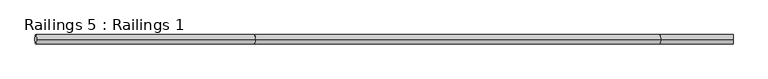
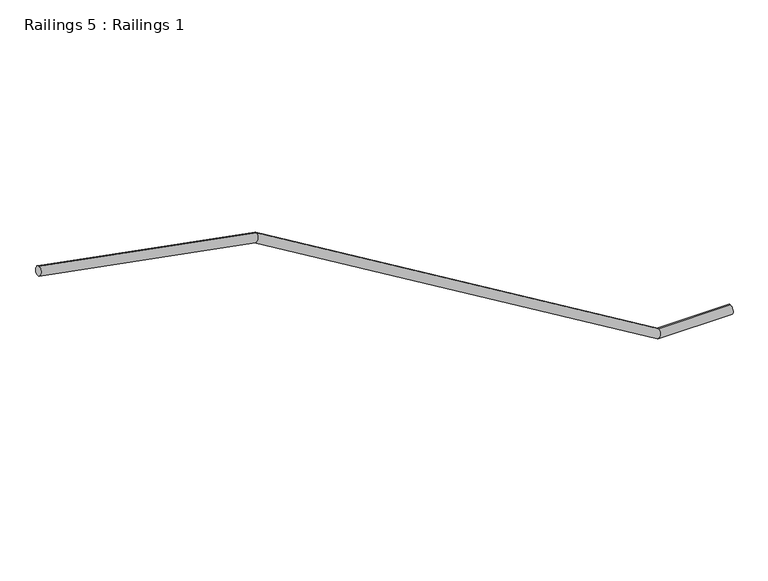
"""IFC4 building model written with IfcOpenShell, lengths in millimetres: railing geometry, Railings 5 : Railings 1."""

from ifc_helpers import new_model, si_unit, frame, origin, place, context, project, spatial, circle_curve, ellipse_curve, source, transform, mapped, element, save
from ifc_brep_helpers import plane_surface, cylinder_surface, advanced_brep


def railings_5_railings_1_26d5b7d0(model_context):
    return source(origin(), model_context, "Body", "AdvancedBrep", [
        advanced_brep(
        [(24288.0514274, 27742.2156612, 266099.6016943), (24281.0618865, 27742.2156612, 266062.1483057), (27167.456657, 27742.2156612, 264922.0), (27167.456657, 27742.2156612, 264883.9), (25193.135822, 27742.2156612, 265930.6950995), (25179.3774919, 27742.2156612, 265894.5049005), (26867.9503269, 27742.2156612, 264922.0), (26857.362987, 27742.2156612, 264883.9)],
        [
            (0, 1, circle_curve(frame((24284.556657, 27742.2156612, 266080.875), z_axis=(-0.9830285726387049, 0.0, 0.18345251531639073), x_axis=(-0.18345251531639073, 0.0, -0.9830285726387049)), 19.05)),
            (1, 0, circle_curve(frame((24284.556657, 27742.2156612, 266080.875), z_axis=(-0.9830285726387049, 0.0, 0.18345251531639073), x_axis=(-0.18345251531639073, 0.0, -0.9830285726387049)), 19.05)),
            (2, 3, circle_curve(frame((27167.456657, 27742.2156612, 264902.95), z_axis=(1.0, 0.0, 0.0), x_axis=(0.0, 0.0, -1.0)), 19.05)),
            (3, 2, circle_curve(frame((27167.456657, 27742.2156612, 264902.95), z_axis=(1.0, 0.0, 0.0), x_axis=(0.0, 0.0, -1.0)), 19.05)),
            (0, 4),
            (4, 5, ellipse_curve(frame((25186.256657, 27742.2156612, 265912.6), z_axis=(-0.9347316453723551, 0.0, 0.3553544021670333), x_axis=(-0.35535440216703496, 0.0, -0.9347316453723546)), 19.3586037, 19.05)),
            (5, 1),
            (5, 4, ellipse_curve(frame((25186.256657, 27742.2156612, 265912.6), z_axis=(-0.9347316453723551, 0.0, 0.3553544021670333), x_axis=(-0.35535440216703496, 0.0, -0.9347316453723546)), 19.3586037, 19.05)),
            (4, 6),
            (6, 7, ellipse_curve(frame((26862.656657, 27742.2156612, 264902.95), z_axis=(-0.9634917766912366, 0.0, 0.2677379245612477), x_axis=(0.26773792456124823, 0.0, 0.9634917766912364)), 19.7718346, 19.05)),
            (7, 5),
            (7, 6, ellipse_curve(frame((26862.656657, 27742.2156612, 264902.95), z_axis=(-0.9634917766912366, 0.0, 0.2677379245612477), x_axis=(0.26773792456124823, 0.0, 0.9634917766912364)), 19.7718346, 19.05)),
            (6, 2),
            (3, 7),
        ],
        [
            plane_surface(frame((24284.556657, 27723.1656612, 266080.875), z_axis=(-0.9830285726387049, 0.0, 0.18345251531639073), x_axis=(0.0, -1.0, 0.0))),
            plane_surface(frame((27167.456657, 27723.1656612, 264902.95), z_axis=(1.0, 0.0, 0.0), x_axis=(0.0, -1.0, 0.0))),
            cylinder_surface(frame((24284.556657, 27742.2156612, 266080.875), z_axis=(-0.9830285726387049, 0.0, 0.18345251531639073), x_axis=(-0.18345251531639073, 0.0, -0.9830285726387049)), 19.05),
            cylinder_surface(frame((25186.256657, 27742.2156612, 265912.6), z_axis=(-0.8566328075032712, 0.0, 0.5159265772462815), x_axis=(-0.5159265772462815, 0.0, -0.8566328075032712)), 19.05),
            cylinder_surface(frame((26862.656657, 27742.2156612, 264902.95), z_axis=(-1.0, 0.0, 0.0), x_axis=(0.0, 0.0, -1.0)), 19.05),
        ],
        [
            (0, [[1, 2]]),
            (1, [[3, 4]]),
            (2, [[-1, 5, 6, 7]]),
            (2, [[-2, -7, 8, -5]]),
            (3, [[-6, 9, 10, 11]]),
            (3, [[-8, -11, 12, -9]]),
            (4, [[-10, 13, -4, 14]]),
            (4, [[-12, -14, -3, -13]]),
        ],
    ),
    ])


if __name__ == "__main__":
    model = new_model("IFC4")
    model_context = context("Model", 3, world=origin())
    ifc_project = project(units=[si_unit("LENGTHUNIT", "METRE", prefix="MILLI")], contexts=[model_context])
    site = spatial("IfcSite", under=ifc_project)
    building = spatial("IfcBuilding", under=site)
    placement = place(None, origin())
    railings_5_railings_1_shape = railings_5_railings_1_26d5b7d0(model_context)
    element("IfcRailing", 1, ObjectType="Railings 5 : Railings 1", at=placement, inside=building, context=model_context, shape_type="MappedRepresentation", body=[
        mapped(railings_5_railings_1_shape, transform((0.0, 0.0, 0.0), x_axis=(1.0, 0.0, 0.0), y_axis=(0.0, 1.0, 0.0), z_axis=(0.0, 0.0, 1.0))),
    ])
    save(model, "model.ifc")

# Revit data of these elements
# Element 1 (IfcRailing, "Railings 5 : Railings 1")
#   Materials on its faces: "ALUM. RAILING"
# Materials
#   "ALUM. RAILING": class "Generic", colour RGB 255 255 255, transparency 0, Cost = 0
